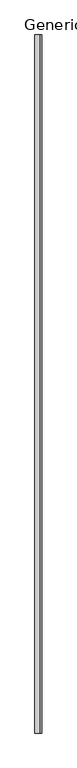
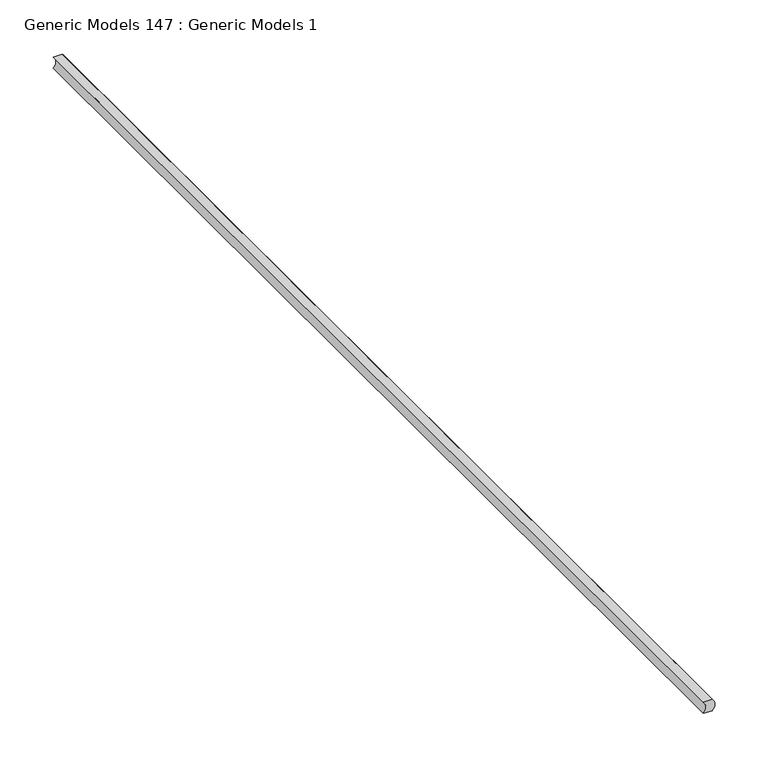
"""IFC4 building model written with IfcOpenShell, lengths in millimetres: proxy geometry, Generic Models 147 : Generic Models 1."""

from ifc_helpers import new_model, si_unit, point, frame, frame_2d, origin, place, context, project, spatial, polyline, circle_curve, trimmed, segment, composite_curve, outline, extrude, source, transform, mapped, element, save


def generic_models_147_generic_models_1_9e68d635(model_context):
    return source(origin(), model_context, "Body", "SweptSolid", [
        extrude(outline(composite_curve([segment(polyline([(2438.4, 50759.2377541), (2438.4, 50768.7627541)]), True, "CONTINUOUS"), segment(trimmed(circle_curve(frame_2d((2444.75, 50762.9332731)), 8.620055), [point((2438.4, 50768.7627541))], [point((2451.1, 50768.7627541))], False, "CARTESIAN"), True, "CONTINUOUS"), segment(polyline([(2451.1, 50768.7627541), (2451.1, 50759.2377541)]), True, "CONTINUOUS"), segment(trimmed(circle_curve(frame_2d((2444.75, 50753.4082731)), 8.620055), [point((2451.1, 50759.2377541))], [point((2438.4, 50759.2377541))], True, "CARTESIAN"), True, "CONTINUOUS")], self_intersect=False)), frame((0.0, 0.0, 0.0), z_axis=(0.0, 1.0, 0.0), x_axis=(0.0, 0.0, 1.0)), (0.0, 0.0, 1.0), 1219.2),
    ])


if __name__ == "__main__":
    model = new_model("IFC4")
    model_context = context("Model", 3, world=origin())
    ifc_project = project(units=[si_unit("LENGTHUNIT", "METRE", prefix="MILLI")], contexts=[model_context])
    site = spatial("IfcSite", under=ifc_project)
    building = spatial("IfcBuilding", under=site)
    placement = place(None, origin())
    generic_models_147_generic_models_1_shape = generic_models_147_generic_models_1_9e68d635(model_context)
    element("IfcBuildingElementProxy", 1, Name="Generic Models 147 : Generic Models 1", ObjectType="Generic Models 147 : Generic Models 1", at=placement, inside=building, context=model_context, shape_type="MappedRepresentation", body=[
        mapped(generic_models_147_generic_models_1_shape, transform((0.0, 0.0, 0.0), x_axis=(1.0, 0.0, 0.0), y_axis=(0.0, 1.0, 0.0), z_axis=(0.0, 0.0, 1.0))),
    ])
    save(model, "model.ifc")

# Revit data of these elements
# Element 1 (IfcBuildingElementProxy, "Generic Models 147 : Generic Models 1")
#   Materials on its faces: "ACOUSTICAL SEALANT"
# Materials
#   "ACOUSTICAL SEALANT": class "Unassigned", colour RGB 120 120 120, transparency 0, Cost = 0
